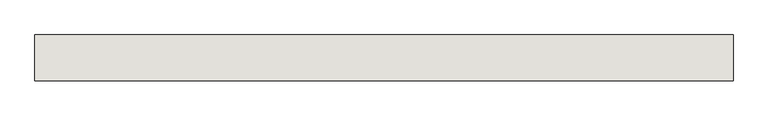
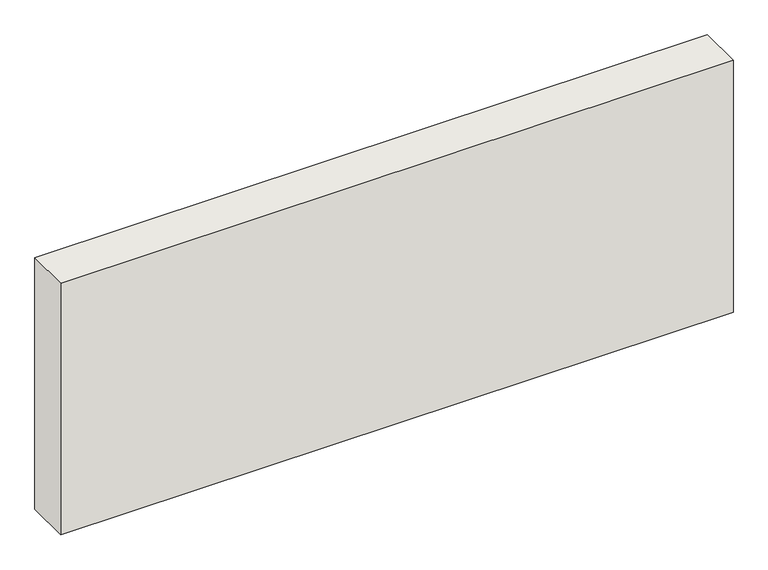
"""IFC4 building model written with IfcOpenShell, lengths in millimetres: wall geometry, Holzwand."""

from ifc_helpers import new_model, si_unit, origin, origin_with_axes, place, context, project, spatial, polyline, outline, extrude, source, transform, mapped, element, save


def wall_f9f172e0(model_context):
    return source(origin(), model_context, "Body", "SweptSolid", [
        extrude(outline(polyline([(0.0, 200.0), (3033.4, 200.0), (3033.4, 0.0), (0.0, 0.0), (0.0, 200.0)])), origin_with_axes(), (0.0, 0.0, 1.0), 1200.0),
    ])


if __name__ == "__main__":
    model = new_model("IFC4")
    model_context = context("Model", 3, world=origin())
    ifc_project = project(units=[si_unit("LENGTHUNIT", "METRE", prefix="MILLI")], contexts=[model_context])
    site = spatial("IfcSite", under=ifc_project)
    building = spatial("IfcBuilding", under=site)
    placement = place(None, origin())
    wall_shape = wall_f9f172e0(model_context)
    element("IfcWall", 1, ObjectType="Holzwand", at=placement, inside=building, context=model_context, shape_type="MappedRepresentation", body=[
        mapped(wall_shape, transform((0.0, 0.0, 0.0), x_axis=(1.0, 0.0, 0.0), y_axis=(0.0, 1.0, 0.0), z_axis=(0.0, 0.0, 1.0))),
    ])
    save(model, "model.ifc")

# Revit data of these elements
# Element 1 (IfcWall, "Holzwand")
#   Materials on its faces: "holzschalung"
# Materials
#   "holzschalung": class "Unassigned", colour RGB 128 128 128, transparency 0
